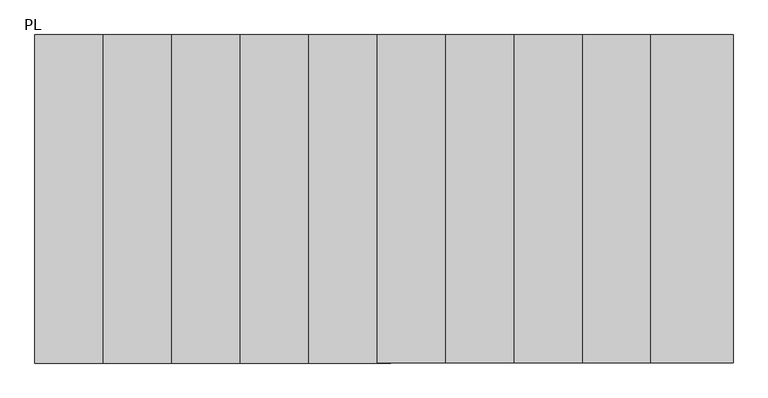
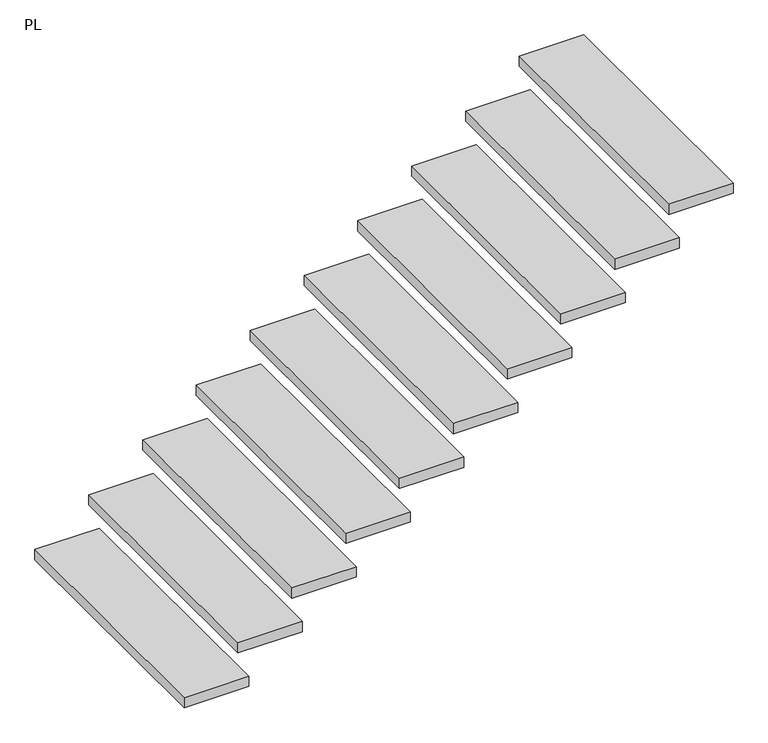
"""IFC4 building model written with IfcOpenShell, lengths in millimetres: stair flight geometry, PL."""

from ifc_helpers import new_model, si_unit, frame, origin, place, context, project, spatial, polyline, outline, extrude, source, transform, mapped, element, save


def pl_d6e87e92(model_context):
    return source(origin(), model_context, "Body", "SweptSolid", [
        extrude(outline(polyline([(4109.5374538, 36032.6086665), (3809.5374538, 36032.6086665), (3809.5374538, 37232.6086665), (4109.5374538, 37232.6086665), (4109.5374538, 36032.6086665)])), frame((0.0, 0.0, 2731.7901873), z_axis=(0.0, 0.0, 1.0), x_axis=(1.0, 0.0, 0.0)), (0.0, 0.0, 1.0), 50.0),
        extrude(outline(polyline([(4359.5374538, 36032.6086665), (4059.5374538, 36032.6086665), (4059.5374538, 37232.6086665), (4359.5374538, 37232.6086665), (4359.5374538, 36032.6086665)])), frame((0.0, 0.0, 2913.6083692), z_axis=(0.0, 0.0, 1.0), x_axis=(1.0, 0.0, 0.0)), (0.0, 0.0, 1.0), 50.0),
        extrude(outline(polyline([(4609.5374538, 36032.6086665), (4309.5374538, 36032.6086665), (4309.5374538, 37232.6086665), (4609.5374538, 37232.6086665), (4609.5374538, 36032.6086665)])), frame((0.0, 0.0, 3095.426551), z_axis=(0.0, 0.0, 1.0), x_axis=(1.0, 0.0, 0.0)), (0.0, 0.0, 1.0), 50.0),
        extrude(outline(polyline([(4859.5374538, 36032.6086665), (4559.5374538, 36032.6086665), (4559.5374538, 37232.6086665), (4859.5374538, 37232.6086665), (4859.5374538, 36032.6086665)])), frame((0.0, 0.0, 3277.2447328), z_axis=(0.0, 0.0, 1.0), x_axis=(1.0, 0.0, 0.0)), (0.0, 0.0, 1.0), 50.0),
        extrude(outline(polyline([(5109.5374538, 36032.6086665), (4809.5374538, 36032.6086665), (4809.5374538, 37232.6086665), (5109.5374538, 37232.6086665), (5109.5374538, 36032.6086665)])), frame((0.0, 0.0, 3459.0629146), z_axis=(0.0, 0.0, 1.0), x_axis=(1.0, 0.0, 0.0)), (0.0, 0.0, 1.0), 50.0),
        extrude(outline(polyline([(5359.5374538, 36032.6086665), (5059.5374538, 36032.6086665), (5059.5374538, 37232.6086665), (5359.5374538, 37232.6086665), (5359.5374538, 36032.6086665)])), frame((0.0, 0.0, 3640.8810964), z_axis=(0.0, 0.0, 1.0), x_axis=(1.0, 0.0, 0.0)), (0.0, 0.0, 1.0), 50.0),
        extrude(outline(polyline([(5609.5374538, 36032.6086665), (5309.5374538, 36032.6086665), (5309.5374538, 37232.6086665), (5609.5374538, 37232.6086665), (5609.5374538, 36032.6086665)])), frame((0.0, 0.0, 3822.6992783), z_axis=(0.0, 0.0, 1.0), x_axis=(1.0, 0.0, 0.0)), (0.0, 0.0, 1.0), 50.0),
        extrude(outline(polyline([(5859.5374538, 36032.6086665), (5559.5374538, 36032.6086665), (5559.5374538, 37232.6086665), (5859.5374538, 37232.6086665), (5859.5374538, 36032.6086665)])), frame((0.0, 0.0, 4004.5174601), z_axis=(0.0, 0.0, 1.0), x_axis=(1.0, 0.0, 0.0)), (0.0, 0.0, 1.0), 50.0),
        extrude(outline(polyline([(6109.5374538, 36032.6086665), (5809.5374538, 36032.6086665), (5809.5374538, 37232.6086665), (6109.5374538, 37232.6086665), (6109.5374538, 36032.6086665)])), frame((0.0, 0.0, 4186.3356419), z_axis=(0.0, 0.0, 1.0), x_axis=(1.0, 0.0, 0.0)), (0.0, 0.0, 1.0), 50.0),
        extrude(outline(polyline([(6359.5374538, 36032.6086665), (6059.5374538, 36032.6086665), (6059.5374538, 37232.6086665), (6359.5374538, 37232.6086665), (6359.5374538, 36032.6086665)])), frame((0.0, 0.0, 4368.1538237), z_axis=(0.0, 0.0, 1.0), x_axis=(1.0, 0.0, 0.0)), (0.0, 0.0, 1.0), 50.0),
    ])


if __name__ == "__main__":
    model = new_model("IFC4")
    model_context = context("Model", 3, world=origin())
    ifc_project = project(units=[si_unit("LENGTHUNIT", "METRE", prefix="MILLI")], contexts=[model_context])
    site = spatial("IfcSite", under=ifc_project)
    building = spatial("IfcBuilding", under=site)
    placement = place(None, origin())
    pl_shape = pl_d6e87e92(model_context)
    element("IfcStairFlight", 1, ObjectType="PL", at=placement, inside=building, context=model_context, shape_type="MappedRepresentation", body=[
        mapped(pl_shape, transform((0.0, 0.0, 0.0), x_axis=(1.0, 0.0, 0.0), y_axis=(0.0, 1.0, 0.0), z_axis=(0.0, 0.0, 1.0))),
    ])
    save(model, "model.ifc")
